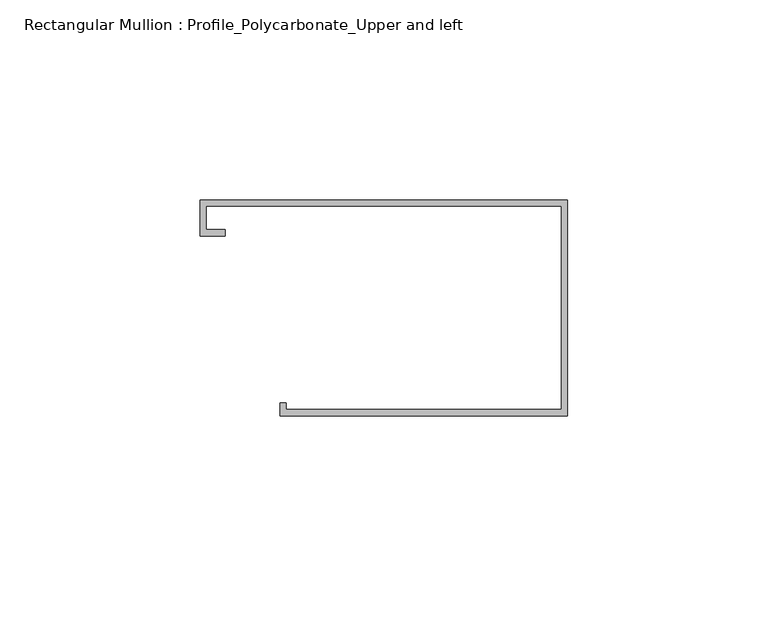
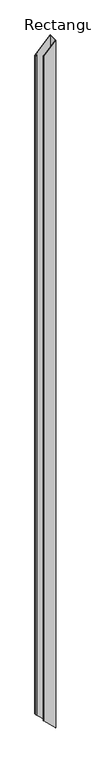
"""IFC4 building model written with IfcOpenShell, lengths in millimetres: member geometry, Rectangular Mullion : Profile_Polycarbonate_Upper and left."""

from ifc_helpers import new_model, si_unit, origin, place, context, project, spatial, faceted_brep, source, transform, mapped, element, save


def rectangular_mullion_profile_polycarbonate_upper_and_left_f746c4a0(model_context):
    return source(origin(), model_context, "Body", "Brep", [
        faceted_brep([(-91.9988, 28.984575, -95.9119088), (0.0, 28.984575, 0.0), (0.0, 28.984575, -4304.390165), (-91.9988, 28.984575, -4216.1448229), (-91.9988, 19.992975, -95.9119088), (-91.9988, 19.992975, -4216.1448229), (-85.6488, 19.992975, -89.2918157), (-85.6488, 19.992975, -4222.2357493), (-85.6488, 21.580475, -89.2918157), (-85.6488, 21.580475, -4222.2357493), (-90.4113, 21.580475, -94.2568855), (-90.4113, 21.580475, -4217.6675545), (-90.4113, 27.397075, -94.2568855), (-90.4113, 27.397075, -4217.6675545), (-1.5875, 27.397075, -1.6550233), (-1.5875, 27.397075, -4302.8674334), (-1.5875, -23.428325, -1.6550233), (-1.5875, -23.428325, -4302.8674334), (-70.3961, -23.428325, -73.3903521), (-70.3961, -23.428325, -4236.8661546), (-70.3961, -21.840825, -73.3903521), (-70.3961, -21.840825, -4236.8661546), (-71.9836, -21.840825, -75.0453753), (-71.9836, -21.840825, -4235.343423), (-71.9836, -25.015825, -75.0453753), (-71.9836, -25.015825, -4235.343423), (0.0, -25.015825, 0.0), (0.0, -25.015825, -4304.390165)], [[[0, 1, 2, 3]], [[4, 0, 3, 5]], [[6, 4, 5, 7]], [[8, 6, 7, 9]], [[10, 8, 9, 11]], [[12, 10, 11, 13]], [[14, 12, 13, 15]], [[16, 14, 15, 17]], [[18, 16, 17, 19]], [[20, 18, 19, 21]], [[22, 20, 21, 23]], [[24, 22, 23, 25]], [[26, 24, 25, 27]], [[1, 26, 27, 2]], [[1, 0, 4, 6, 8, 10, 12, 14, 16, 18, 20, 22, 24, 26]], [[2, 27, 25, 23, 21, 19, 17, 15, 13, 11, 9, 7, 5, 3]]]),
    ])


if __name__ == "__main__":
    model = new_model("IFC4")
    model_context = context("Model", 3, world=origin())
    ifc_project = project(units=[si_unit("LENGTHUNIT", "METRE", prefix="MILLI")], contexts=[model_context])
    site = spatial("IfcSite", under=ifc_project)
    building = spatial("IfcBuilding", under=site)
    placement = place(None, origin())
    rectangular_mullion_profile_polycarbonate_upper_and_left_shape = rectangular_mullion_profile_polycarbonate_upper_and_left_f746c4a0(model_context)
    element("IfcMember", 1, ObjectType="Rectangular Mullion : Profile_Polycarbonate_Upper and left", at=placement, inside=building, context=model_context, shape_type="MappedRepresentation", body=[
        mapped(rectangular_mullion_profile_polycarbonate_upper_and_left_shape, transform((0.0, 0.0, 0.0), x_axis=(1.0, 0.0, 0.0), y_axis=(0.0, 1.0, 0.0), z_axis=(0.0, 0.0, 1.0))),
    ])
    save(model, "model.ifc")

# Revit data of these elements
# Type "Rectangular Mullion : Profile_Polycarbonate_Upper and left"
#   built-in parameter 1007322 = 0.177167 (stored number, unit not read)
#   built-in parameter 1007321 = 0.00520833 (stored number, unit not read)
#   built-in parameter 1007320 = 0 (stored number, unit not read)
